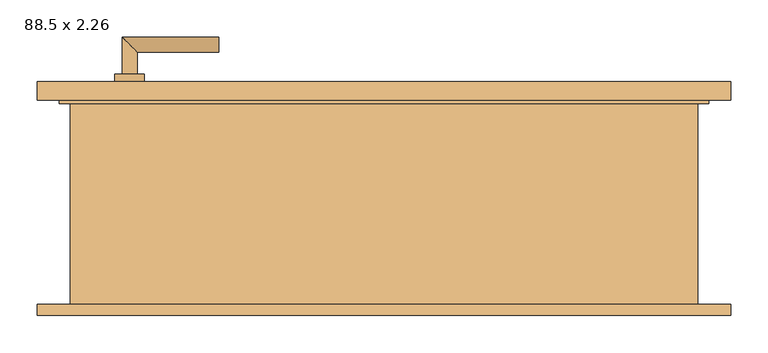
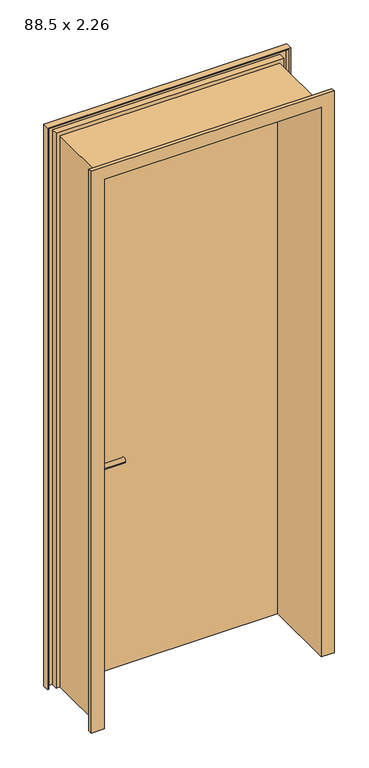
"""IFC4 building model written with IfcOpenShell, lengths in millimetres: door geometry, Drehflügel 1-flg - Stahlzarge : 88.5 x 2.26."""

from ifc_helpers import new_model, si_unit, point, frame, frame_2d, origin, place, context, project, spatial, polyline, circle_curve, ellipse_curve, trimmed, segment, composite_curve, outline, extrude, faceted_brep, source, transform, mapped, element, save
from ifc_brep_helpers import plane_surface, cylinder_surface, advanced_brep


def door_88_5_x_2_26_ebc13128(model_context):
    return source(origin(), model_context, "Body", "SolidModel", [
        advanced_brep(
        [(-352.5, 126.9346141, 1000.0), (-332.5, 126.9346141, 1000.0), (-352.5, 56.9346141, 1000.0), (-332.5, 76.9346141, 1000.0), (-222.5, 56.9346141, 1000.0), (-222.5, 76.9346141, 1000.0)],
        [
            (0, 1, circle_curve(frame((-342.5, 126.9346141, 1000.0), z_axis=(0.0, 1.0, 0.0), x_axis=(1.0, 0.0, 0.0)), 10.0)),
            (1, 0, circle_curve(frame((-342.5, 126.9346141, 1000.0), z_axis=(0.0, 1.0, 0.0), x_axis=(1.0, 0.0, 0.0)), 10.0)),
            (0, 2),
            (2, 3, ellipse_curve(frame((-342.5, 66.9346141, 1000.0), z_axis=(-0.7071067811865385, 0.7071067811865565, 0.0), x_axis=(0.7071067811865563, 0.7071067811865386, 0.0)), 14.1421356, 10.0)),
            (3, 1),
            (3, 2, ellipse_curve(frame((-342.5, 66.9346141, 1000.0), z_axis=(-0.7071067811865385, 0.7071067811865565, 0.0), x_axis=(0.7071067811865563, 0.7071067811865386, 0.0)), 14.1421356, 10.0)),
            (4, 5, circle_curve(frame((-222.5, 66.9346141, 1000.0), z_axis=(1.0, 0.0, 0.0), x_axis=(0.0, 1.0, 0.0)), 10.0)),
            (5, 4, circle_curve(frame((-222.5, 66.9346141, 1000.0), z_axis=(1.0, 0.0, 0.0), x_axis=(0.0, 1.0, 0.0)), 10.0)),
            (2, 4),
            (5, 3),
        ],
        [
            plane_surface(frame((-342.5, 126.9346141, -287.7526403), z_axis=(0.0, 1.0, 0.0), x_axis=(0.0, 0.0, 1.0))),
            cylinder_surface(frame((-342.5, 126.9346141, 1000.0), z_axis=(0.0, 1.0, 0.0), x_axis=(1.0, 0.0, 0.0)), 10.0),
            plane_surface(frame((-222.5, 66.9346141, -287.7526403), z_axis=(1.0, 0.0, 0.0), x_axis=(0.0, 0.0, 1.0))),
            cylinder_surface(frame((-342.5, 66.9346141, 1000.0), z_axis=(-1.0, 0.0, 0.0), x_axis=(0.0, 1.0, 0.0)), 10.0),
        ],
        [
            (0, [[1, 2]]),
            (1, [[-1, 3, 4, 5]]),
            (1, [[-2, -5, 6, -3]]),
            (2, [[7, 8]]),
            (3, [[-4, 9, -8, 10]]),
            (3, [[-6, -10, -7, -9]]),
        ],
    ),
        advanced_brep(
        [(-332.5, 186.9346141, 1000.0), (-352.5, 186.9346141, 1000.0), (-332.5, 216.9346141, 1000.0), (-352.5, 236.9346141, 1000.0), (-222.5, 216.9346141, 1000.0), (-222.5, 236.9346141, 1000.0)],
        [
            (0, 1, circle_curve(frame((-342.5, 186.9346141, 1000.0), z_axis=(0.0, -1.0, 0.0), x_axis=(-1.0, 0.0, 0.0)), 10.0)),
            (1, 0, circle_curve(frame((-342.5, 186.9346141, 1000.0), z_axis=(0.0, -1.0, 0.0), x_axis=(-1.0, 0.0, 0.0)), 10.0)),
            (0, 2),
            (2, 3, ellipse_curve(frame((-342.5, 226.9346141, 1000.0), z_axis=(-0.7071067811865475, -0.7071067811865475, 0.0), x_axis=(0.7071067811865474, -0.7071067811865476, 0.0)), 14.1421356, 10.0)),
            (3, 1),
            (3, 2, ellipse_curve(frame((-342.5, 226.9346141, 1000.0), z_axis=(-0.7071067811865475, -0.7071067811865475, 0.0), x_axis=(0.7071067811865474, -0.7071067811865476, 0.0)), 14.1421356, 10.0)),
            (4, 5, circle_curve(frame((-222.5, 226.9346141, 1000.0), z_axis=(1.0, 0.0, 0.0), x_axis=(0.0, 1.0, 0.0)), 10.0)),
            (5, 4, circle_curve(frame((-222.5, 226.9346141, 1000.0), z_axis=(1.0, 0.0, 0.0), x_axis=(0.0, 1.0, 0.0)), 10.0)),
            (2, 4),
            (5, 3),
        ],
        [
            plane_surface(frame((-342.5, 186.9346141, -287.7526403), z_axis=(0.0, -1.0, 0.0), x_axis=(0.0, 0.0, 1.0))),
            cylinder_surface(frame((-342.5, 186.9346141, 1000.0), z_axis=(0.0, -1.0, 0.0), x_axis=(-1.0, 0.0, 0.0)), 10.0),
            plane_surface(frame((-222.5, 226.9346141, -287.7526403), z_axis=(1.0, 0.0, 0.0), x_axis=(0.0, 0.0, 1.0))),
            cylinder_surface(frame((-342.5, 226.9346141, 1000.0), z_axis=(-1.0, 0.0, 0.0), x_axis=(0.0, 1.0, 0.0)), 10.0),
        ],
        [
            (0, [[1, 2]]),
            (1, [[-1, 3, 4, 5]]),
            (1, [[-2, -5, 6, -3]]),
            (2, [[7, 8]]),
            (3, [[-4, 9, -8, 10]]),
            (3, [[-6, -10, -7, -9]]),
        ],
    ),
        extrude(outline(composite_curve([segment(trimmed(circle_curve(frame_2d((1000.0, -342.5)), 20.0), [point((1000.0, -362.5))], [point((1000.0, -322.5))], False, "CARTESIAN"), True, "CONTINUOUS"), segment(trimmed(circle_curve(frame_2d((1000.0, -342.5)), 20.0), [point((1000.0, -322.5))], [point((1000.0, -362.5))], False, "CARTESIAN"), True, "CONTINUOUS")], self_intersect=False)), frame((0.0, 116.9346141, 0.0), z_axis=(0.0, 1.0, 0.0), x_axis=(0.0, 0.0, 1.0)), (0.0, 0.0, 1.0), 10.0),
        extrude(outline(composite_curve([segment(trimmed(circle_curve(frame_2d((1000.0, -342.5)), 20.0), [point((1000.0, -362.5))], [point((1000.0, -322.5))], False, "CARTESIAN"), True, "CONTINUOUS"), segment(trimmed(circle_curve(frame_2d((1000.0, -342.5)), 20.0), [point((1000.0, -322.5))], [point((1000.0, -362.5))], False, "CARTESIAN"), True, "CONTINUOUS")], self_intersect=False)), frame((0.0, 176.9346141, 0.0), z_axis=(0.0, 1.0, 0.0), x_axis=(0.0, 0.0, 1.0)), (0.0, 0.0, 1.0), 10.0),
        extrude(outline(polyline([(432.5, 151.9346141), (-432.5, 151.9346141), (-432.5, 176.9346141), (432.5, 176.9346141), (432.5, 151.9346141)])), frame((0.0, 0.0, 100.0), z_axis=(0.0, 0.0, 1.0), x_axis=(1.0, 0.0, 0.0)), (0.0, 0.0, 1.0), 2250.0),
        faceted_brep([(466.9603207, -138.0653859, 100.0), (417.5, -138.0653859, 100.0), (417.5, 151.9346141, 100.0), (432.5, 151.9346141, 100.0), (432.5, 176.9346141, 100.0), (466.9603207, 176.9346141, 100.0), (466.9603207, 151.9346141, 100.0), (461.9603207, 151.9346141, 100.0), (461.9603207, 171.9346141, 100.0), (437.5, 171.9346141, 100.0), (437.5, 146.9346141, 100.0), (422.5, 146.9346141, 100.0), (422.5, -133.0653859, 100.0), (461.9603207, -133.0653859, 100.0), (461.9603207, -123.0653859, 100.0), (466.9603207, -123.0653859, 100.0), (466.9603207, -138.0653859, 2384.4603207), (-466.9603207, -138.0653859, 2384.4603207), (-466.9603207, -138.0653859, 100.0), (-417.5, -138.0653859, 100.0), (-417.5, -138.0653859, 2335.0), (417.5, -138.0653859, 2335.0), (417.5, 151.9346141, 2335.0), (-417.5, 151.9346141, 2335.0), (-417.5, 151.9346141, 100.0), (-432.5, 151.9346141, 100.0), (-432.5, 151.9346141, 2350.0), (432.5, 151.9346141, 2350.0), (432.5, 176.9346141, 2350.0), (-432.5, 176.9346141, 2350.0), (-432.5, 176.9346141, 100.0), (-466.9603207, 176.9346141, 100.0), (-466.9603207, 176.9346141, 2384.4603207), (466.9603207, 176.9346141, 2384.4603207), (466.9603207, 151.9346141, 2384.4603207), (-466.9603207, 151.9346141, 2384.4603207), (-466.9603207, 151.9346141, 100.0), (-461.9603207, 151.9346141, 100.0), (-461.9603207, 151.9346141, 2379.4603207), (461.9603207, 151.9346141, 2379.4603207), (461.9603207, 171.9346141, 2379.4603207), (-461.9603207, 171.9346141, 2379.4603207), (-461.9603207, 171.9346141, 100.0), (-437.5, 171.9346141, 100.0), (-437.5, 171.9346141, 2355.0), (437.5, 171.9346141, 2355.0), (437.5, 146.9346141, 2355.0), (-437.5, 146.9346141, 2355.0), (-437.5, 146.9346141, 100.0), (-422.5, 146.9346141, 100.0), (-422.5, 146.9346141, 2340.0), (422.5, 146.9346141, 2340.0), (422.5, -133.0653859, 2340.0), (-422.5, -133.0653859, 2340.0), (-422.5, -133.0653859, 100.0), (-461.9603207, -133.0653859, 100.0), (-461.9603207, -133.0653859, 2379.4603207), (461.9603207, -133.0653859, 2379.4603207), (461.9603207, -123.0653859, 2379.4603207), (-461.9603207, -123.0653859, 2379.4603207), (-461.9603207, -123.0653859, 100.0), (-466.9603207, -123.0653859, 100.0), (-466.9603207, -123.0653859, 2384.4603207), (466.9603207, -123.0653859, 2384.4603207)], [[[0, 1, 2, 3, 4, 5, 6, 7, 8, 9, 10, 11, 12, 13, 14, 15]], [[1, 0, 16, 17, 18, 19, 20, 21]], [[2, 1, 21, 22]], [[3, 2, 22, 23, 24, 25, 26, 27]], [[4, 3, 27, 28]], [[5, 4, 28, 29, 30, 31, 32, 33]], [[6, 5, 33, 34]], [[7, 6, 34, 35, 36, 37, 38, 39]], [[8, 7, 39, 40]], [[9, 8, 40, 41, 42, 43, 44, 45]], [[10, 9, 45, 46]], [[11, 10, 46, 47, 48, 49, 50, 51]], [[12, 11, 51, 52]], [[13, 12, 52, 53, 54, 55, 56, 57]], [[14, 13, 57, 58]], [[15, 14, 58, 59, 60, 61, 62, 63]], [[0, 15, 63, 16]], [[17, 62, 61, 18]], [[18, 61, 60, 55, 54, 49, 48, 43, 42, 37, 36, 31, 30, 25, 24, 19]], [[23, 20, 19, 24]], [[29, 26, 25, 30]], [[35, 32, 31, 36]], [[41, 38, 37, 42]], [[47, 44, 43, 48]], [[53, 50, 49, 54]], [[59, 56, 55, 60]], [[22, 21, 20, 23]], [[28, 27, 26, 29]], [[34, 33, 32, 35]], [[40, 39, 38, 41]], [[46, 45, 44, 47]], [[52, 51, 50, 53]], [[58, 57, 56, 59]], [[16, 63, 62, 17]]]),
    ])


if __name__ == "__main__":
    model = new_model("IFC4")
    model_context = context("Model", 3, world=origin())
    ifc_project = project(units=[si_unit("LENGTHUNIT", "METRE", prefix="MILLI")], contexts=[model_context])
    site = spatial("IfcSite", under=ifc_project)
    building = spatial("IfcBuilding", under=site)
    placement = place(None, origin())
    door_88_5_x_2_26_shape = door_88_5_x_2_26_ebc13128(model_context)
    element("IfcDoor", 1, ObjectType="Drehflügel 1-flg - Stahlzarge : 88.5 x 2.26", at=placement, inside=building, context=model_context, shape_type="MappedRepresentation", body=[
        mapped(door_88_5_x_2_26_shape, transform((0.0, 0.0, 0.0), x_axis=(1.0, 0.0, 0.0), y_axis=(0.0, 1.0, 0.0), z_axis=(0.0, 0.0, 1.0))),
    ])
    save(model, "model.ifc")

# Revit data of these elements
# Type "Drehflügel 1-flg - Stahlzarge : 88.5 x 2.26"
#   Type Mark = "21"
#   Operation = "SingleSwingRight"
#   Keynote = "16.03"
#   Analytic Construction = "Metall"
#   Thermal Resistance (R) = 0.270117 (m²·K)/W
#   Heat Transfer Coefficient (U) = 3.7021 W/(m²·K)
#   Rough Width = 0.885 m
#   Rough Height [instance default] = 2.360 m
#   Höhe Türgriff [instance default] = 0.900 m
#   Height = 2.260 m
#   Fußbodenaufbau [instance default] = 0.100 m
#   Width = 0.885 m
#   Sichtbarkeit Sturzlinien [instance default] = yes
#   Türgriff auswählen [instance default] = element 221079
#   Türgriff [instance default] = none
#   Türflügel [instance default] = none
#   Rahmen/Pfosten [instance default] = Metall - Lackiert - Grau
#   Visual Light Transmittance = 0
#   Solar Heat Gain Coefficient = 0
#   Function = (empty or 0)
#   Wall Closure = (empty or 0)
# Element 1 (IfcDoor, "Drehflügel 1-flg - Stahlzarge : 88.5 x 2.26")
#   Materials on its faces: "Metall - Lackiert - Grau", "Metall - Chrom", "Holz - Birke"
# Materials
#   "Metall - Lackiert - Grau": class "Farbe 1", colour RGB 98 98 98, transparency 0, Cost = 0
#   "Metall - Chrom": class "Metall", colour RGB 247 247 247, transparency 0, Cost = 0
#   "Holz - Birke": class "Holz", colour RGB 213 164 103, transparency 0, Cost = 0
